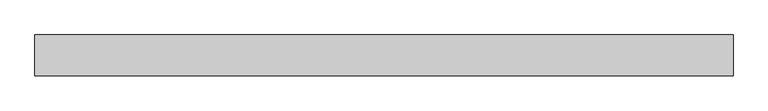
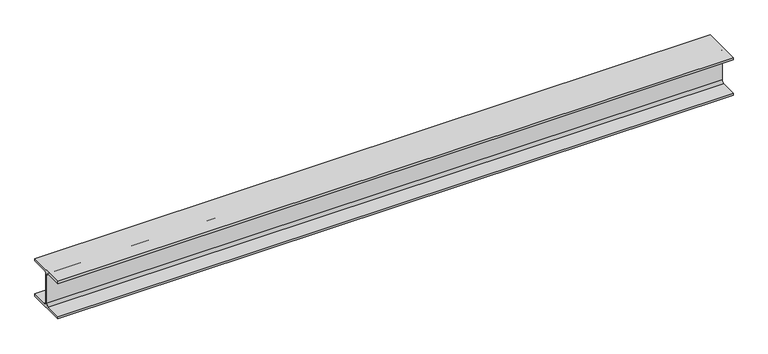
"""IFC4 building model written with IfcOpenShell, lengths in millimetres: beam geometry, 0912_Steel Framing_H-KSD3502 : H_SB_ASB_H-200x200x8x12."""

from ifc_helpers import new_model, si_unit, point, frame, frame_2d, origin, place, context, project, spatial, polyline, circle_curve, trimmed, segment, composite_curve, outline, extrude, source, transform, mapped, element, save


def beam_623e387b(model_context):
    return source(origin(), model_context, "Body", "SweptSolid", [
        extrude(outline(composite_curve([segment(polyline([(-100.0, -88.0), (-17.0, -88.0)]), True, "CONTINUOUS"), segment(trimmed(circle_curve(frame_2d((-17.0, -75.0)), 13.0), [point((-17.0, -88.0))], [point((-4.0, -75.0))], True, "CARTESIAN"), True, "CONTINUOUS"), segment(polyline([(-4.0, -75.0), (-4.0, 75.0)]), True, "CONTINUOUS"), segment(trimmed(circle_curve(frame_2d((-17.0, 75.0)), 13.0), [point((-4.0, 75.0))], [point((-17.0, 88.0))], True, "CARTESIAN"), True, "CONTINUOUS"), segment(polyline([(-17.0, 88.0), (-100.0, 88.0), (-100.0, 100.0), (100.0, 100.0), (100.0, 88.0), (17.0, 88.0)]), True, "CONTINUOUS"), segment(trimmed(circle_curve(frame_2d((17.0, 75.0)), 13.0), [point((17.0, 88.0))], [point((4.0, 75.0))], True, "CARTESIAN"), True, "CONTINUOUS"), segment(polyline([(4.0, 75.0), (4.0, -75.0)]), True, "CONTINUOUS"), segment(trimmed(circle_curve(frame_2d((17.0, -75.0)), 13.0), [point((4.0, -75.0))], [point((17.0, -88.0))], True, "CARTESIAN"), True, "CONTINUOUS"), segment(polyline([(17.0, -88.0), (100.0, -88.0), (100.0, -100.0), (-100.0, -100.0), (-100.0, -88.0)]), True, "CONTINUOUS")], self_intersect=False)), frame((-1715.1887846, 0.0, 0.0), z_axis=(1.0, 0.0, 0.0), x_axis=(0.0, 1.0, 0.0)), (0.0, 0.0, 1.0), 3399.973917),
    ])


if __name__ == "__main__":
    model = new_model("IFC4")
    model_context = context("Model", 3, world=origin())
    ifc_project = project(units=[si_unit("LENGTHUNIT", "METRE", prefix="MILLI")], contexts=[model_context])
    site = spatial("IfcSite", under=ifc_project)
    building = spatial("IfcBuilding", under=site)
    placement = place(None, origin())
    beam_shape = beam_623e387b(model_context)
    element("IfcBeam", 1, ObjectType="0912_Steel Framing_H-KSD3502 : H_SB_ASB_H-200x200x8x12", at=placement, inside=building, context=model_context, shape_type="MappedRepresentation", body=[
        mapped(beam_shape, transform((0.0, 0.0, 0.0), x_axis=(1.0, 0.0, 0.0), y_axis=(0.0, 1.0, 0.0), z_axis=(0.0, 0.0, 1.0))),
    ])
    save(model, "model.ifc")

# Revit data of these elements
# Type "0912_Steel Framing_H-KSD3502 : H_SB_ASB_H-200x200x8x12"
#   H_WM Code_1 = "S01AA002-00001 | Main Steel Structure Fabrication Work | Shelter/Building | Medium Steel - Standard (90KG/M>Weight≥30KG/M) | Material: (   )"
#   H_WM Code_2 = "S03AA028-00001 | Main Steel Structure Erection Work | Shelter/Building | Medium Steel (90KG/M>Weight≥30KG/M) | Material: (   )"
#   H_WM Code_3 = "S01AA010-00001 | Main Steel Structure Fabrication Work | Shelter/Building | Steel Painting/Coating | for Non-Fireproofed Steel Surface, Surface Preparation, Primer, Second & Final Coat | Material: (   )"
#   H_Q'ty Cal Type Tag = "SB-Q2"
#   Width = 20.0 cm
#   Web Thickness = 0.8 cm
#   Web Fillet = 1.3 cm
#   Warping Constant = 141000.0 cm⁶
#   W = 0
#   Torsional Moment of Inertia = 26.2485 cm⁴
#   Section Area = 63.53 cm²
#   Plastic Modulus weak axis = 244.0 cm³
#   Plastic Modulus strong axis = 525.0 cm³
#   Perimeter = 1.16 m²/m
#   Nominal Weight = 49.90 kgf/m
#   Moment of Inertia weak axis = 1600.00 cm⁴
#   Moment of Inertia strong axis = 4720.00 cm⁴
#   Height = 20.0 cm
#   Flange Thickness = 1.2 cm
#   Elastic Modulus weak axis = 160.0 cm³
#   Elastic Modulus strong axis = 472.0 cm³
#   Centroid Vertical = 10.0 cm
#   Centroid Horizontal = 10.0 cm
#   Ix = 47200000
#   Length [instance default] = 1.5240 m
#   Zx = 525000
#   b = 0.2000 m
#   h = 0.2000 m
#   r = 0.0130 m
#   s = 0.0080 m
#   t = 0.0120 m
#   A = 0.006353 m²
#   Structural Material [instance default] = Steel, 45-345
#   Assembly Code = ""
# Element 1 (IfcBeam, "0912_Steel Framing_H-KSD3502 : H_SB_ASB_H-200x200x8x12")
#   Structural Material = none
# Materials
#   "Steel, 45-345": class "Metal", colour RGB 189 187 185, transparency 0, Description = "Steel 345 MPa", Cost = 0
